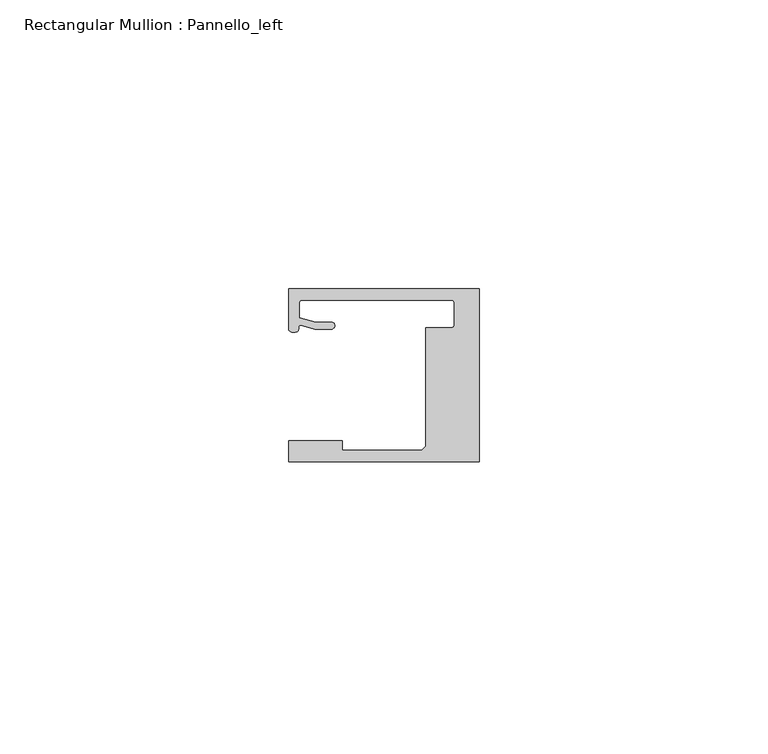
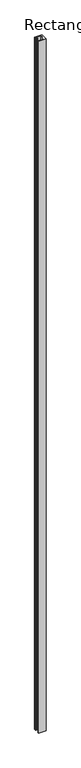
"""IFC4 building model written with IfcOpenShell, lengths in millimetres: member geometry, Rectangular Mullion : Pannello_left."""

from ifc_helpers import new_model, si_unit, frame, origin, place, context, project, spatial, polyline, circle_curve, source, transform, mapped, element, save
from ifc_brep_helpers import plane_surface, cylinder_surface, revolved_surface, extruded_surface, spline_curve, advanced_brep


def rectangular_mullion_pannello_left_2a30ab1a(model_context):
    return source(origin(), model_context, "Body", "AdvancedBrep", [
        advanced_brep(
        [(-33.0, -15.0, 0.0), (0.0, -15.0, 0.0), (0.0, 15.0, 0.0), (-33.0000135, 15.0, 0.0), (-33.0000135, 8.0000472, 0.0), (-30.9223017, 8.6490241, 0.0), (-28.4999305, 7.9999523, 0.0), (-25.59998, 7.9999523, 0.0), (-25.59998, 9.1999523, 0.0), (-28.3419477, 9.1999523, 0.0), (-31.19998, 9.9657591, 0.0), (-31.19998, 12.50001, 0.0), (-30.69998, 13.00001, 0.0), (-4.7999726, 13.00001, 0.0), (-4.2999726, 12.50001, 0.0), (-4.2999726, 8.7500595, 0.0), (-4.7999726, 8.2500595, 0.0), (-9.2999726, 8.2500595, 0.0), (-9.2999726, -12.2999849, 0.0), (-10.0000103, -13.0000004, 0.0), (-23.700041, -13.0000004, 0.0), (-23.700041, -11.3000004, 0.0), (-33.0, -11.3000004, 0.0), (-33.0, -15.0, -3248.9999865), (-33.0, -11.3000004, -3248.9999865), (-23.700041, -11.3000004, -3248.9999865), (-23.700041, -13.0000004, -3248.9999865), (-10.0000103, -13.0000004, -3248.9999865), (-9.2999726, -12.2999849, -3248.9999865), (-9.2999726, 8.2500595, -3248.9999865), (-4.7999726, 8.2500595, -3248.9999865), (-4.2999726, 8.7500595, -3248.9999865), (-4.2999726, 12.50001, -3248.9999865), (-4.7999726, 13.00001, -3248.9999865), (-30.69998, 13.00001, -3248.9999865), (-31.19998, 12.50001, -3248.9999865), (-31.19998, 9.9657591, -3248.9999865), (-28.3419477, 9.1999523, -3248.9999865), (-25.59998, 9.1999523, -3248.9999865), (-25.59998, 7.9999523, -3248.9999865), (-28.4999305, 7.9999523, -3248.9999865), (-30.9223017, 8.6490241, -3248.9999865), (-33.0000135, 8.0000472, -3248.9999865), (-33.0000135, 15.0, -3248.9999865), (0.0, 15.0, -3248.9999865), (0.0, -15.0, -3248.9999865)],
        [
            (0, 1),
            (1, 2),
            (2, 3),
            (3, 4),
            (4, 5, spline_curve(3, [(-33.0000135, 8.0000472, 0.0), (-33.0000135, 7.457047519, 0.0), (-32.262327879, 7.456527435, 0.0), (-31.357433266, 7.563996614, 0.0), (-31.305645054, 7.690065204, 0.0), (-31.298563602, 8.366228555, 0.0), (-31.312054066, 8.717747958, 0.0), (-30.9223017, 8.6490241, 0.0)], [4, 2, 2, 4], [0.0, 0.0027053965905959043, 0.0058611956533709, 0.007702013405570312])),
            (5, 6),
            (6, 7),
            (7, 8, circle_curve(frame((-25.59998, 8.5999523, 0.0), z_axis=(0.0, 0.0, 1.0), x_axis=(0.0, 1.0, 0.0)), 0.6)),
            (8, 9),
            (9, 10),
            (10, 11),
            (11, 12, circle_curve(frame((-30.69998, 12.50001, 0.0), z_axis=(0.0, 0.0, -1.0), x_axis=(0.0, 1.0, 0.0)), 0.5)),
            (12, 13),
            (13, 14, circle_curve(frame((-4.7999726, 12.50001, 0.0), z_axis=(0.0, 0.0, -1.0), x_axis=(1.0, 0.0, 0.0)), 0.5)),
            (14, 15),
            (15, 16, circle_curve(frame((-4.7999726, 8.7500595, 0.0), z_axis=(0.0, 0.0, -1.0), x_axis=(0.0, -1.0, 0.0)), 0.5)),
            (16, 17),
            (17, 18),
            (18, 19),
            (19, 20),
            (20, 21),
            (21, 22),
            (22, 0),
            (23, 24),
            (24, 25),
            (25, 26),
            (26, 27),
            (27, 28),
            (28, 29),
            (29, 30),
            (30, 31, circle_curve(frame((-4.7999726, 8.7500595, -3248.9999865), z_axis=(0.0, 0.0, 1.0), x_axis=(0.0, -1.0, 0.0)), 0.5)),
            (31, 32),
            (32, 33, circle_curve(frame((-4.7999726, 12.50001, -3248.9999865), z_axis=(0.0, 0.0, 1.0), x_axis=(1.0, 0.0, 0.0)), 0.5)),
            (33, 34),
            (34, 35, circle_curve(frame((-30.69998, 12.50001, -3248.9999865), z_axis=(0.0, 0.0, 1.0), x_axis=(0.0, 1.0, 0.0)), 0.5)),
            (35, 36),
            (36, 37),
            (37, 38),
            (38, 39, circle_curve(frame((-25.59998, 8.5999523, -3248.9999865), z_axis=(0.0, 0.0, -1.0), x_axis=(0.0, 1.0, 0.0)), 0.6)),
            (39, 40),
            (40, 41),
            (41, 42, spline_curve(3, [(-30.9223017, 8.6490241, -3248.9999865), (-31.312054066, 8.717747958, -3248.9999865), (-31.298563602, 8.366228555, -3248.9999865), (-31.305645054, 7.690065204, -3248.9999865), (-31.357433266, 7.563996614, -3248.9999865), (-32.262327879, 7.456527435, -3248.9999865), (-33.0000135, 7.457047519, -3248.9999865), (-33.0000135, 8.0000472, -3248.9999865)], [4, 2, 2, 4], [0.0, 0.001840817752199412, 0.004996616814974408, 0.007702013405570312])),
            (42, 43),
            (43, 44),
            (44, 45),
            (45, 23),
            (0, 23),
            (45, 1),
            (44, 2),
            (43, 3),
            (42, 4),
            (41, 5),
            (40, 6),
            (39, 7),
            (38, 8),
            (37, 9),
            (36, 10),
            (35, 11),
            (34, 12),
            (33, 13),
            (32, 14),
            (31, 15),
            (30, 16),
            (29, 17),
            (28, 18),
            (27, 19),
            (26, 20),
            (25, 21),
            (24, 22),
        ],
        [
            plane_surface(frame((0.0, -36.2491502, 0.0), z_axis=(0.0, 0.0, 1.0), x_axis=(-1.0, 0.0, 0.0))),
            plane_surface(frame((0.0, -36.2491502, -3248.9999865), z_axis=(0.0, 0.0, -1.0), x_axis=(-1.0, 0.0, 0.0))),
            plane_surface(frame((-33.0, -15.0, 0.0), z_axis=(0.0, -1.0, 0.0), x_axis=(0.0, 0.0, -1.0))),
            plane_surface(frame((0.0, -15.0, 0.0), z_axis=(1.0, 0.0, 0.0), x_axis=(0.0, 0.0, -1.0))),
            plane_surface(frame((0.0, 15.0, 0.0), z_axis=(0.0, 1.0, 0.0), x_axis=(0.0, 0.0, -1.0))),
            plane_surface(frame((-33.0000135, 15.0, 0.0), z_axis=(-1.0, 0.0, 0.0), x_axis=(0.0, 0.0, -1.0))),
            extruded_surface(spline_curve(3, [(-33.0000135, 8.0000472, -3248.9999865), (-33.0000135, 7.457047519, -3248.9999865), (-32.262327879, 7.456527435, -3248.9999865), (-31.357433266, 7.563996614, -3248.9999865), (-31.305645054, 7.690065204, -3248.9999865), (-31.298563602, 8.366228555, -3248.9999865), (-31.312054066, 8.717747958, -3248.9999865), (-30.9223017, 8.6490241, -3248.9999865)], [4, 2, 2, 4], [0.0, 0.0027053965905959043, 0.0058611956533709, 0.007702013405570312]), (0.0, 0.0, 3248.9999865), 3248.9999865),
            plane_surface(frame((-30.9223017, 8.6490241, 0.0), z_axis=(-0.25881883200192934, -0.9659258833891746, 0.0), x_axis=(0.0, 0.0, -1.0))),
            plane_surface(frame((-28.4999305, 7.9999523, 0.0), z_axis=(0.0, -1.0, 0.0), x_axis=(0.0, 0.0, -1.0))),
            cylinder_surface(frame((-25.59998, 8.5999523, 0.0), z_axis=(0.0, 0.0, 1.0), x_axis=(0.0, 1.0, 0.0)), 0.6),
            plane_surface(frame((-25.59998, 9.1999523, 0.0), z_axis=(0.0, 1.0, 0.0), x_axis=(0.0, 0.0, -1.0))),
            plane_surface(frame((-28.3419477, 9.1999523, 0.0), z_axis=(0.25881883204288636, 0.9659258833782002, 0.0), x_axis=(0.0, 0.0, -1.0))),
            plane_surface(frame((-31.19998, 9.9657591, 0.0), z_axis=(1.0, 0.0, 0.0), x_axis=(0.0, 0.0, -1.0))),
            revolved_surface(polyline([(-30.69998, 13.00001, -3248.9999865), (-30.69998, 13.00001, 0.0)]), (-30.69998, 12.50001, 0.0), (0.0, 0.0, -1.0)),
            plane_surface(frame((-30.69998, 13.00001, 0.0), z_axis=(0.0, -1.0, 0.0), x_axis=(0.0, 0.0, -1.0))),
            revolved_surface(polyline([(-4.2999726, 12.50001, -3248.9999865), (-4.2999726, 12.50001, 0.0)]), (-4.7999726, 12.50001, 0.0), (0.0, 0.0, -1.0)),
            plane_surface(frame((-4.2999726, 12.50001, 0.0), z_axis=(-1.0, 0.0, 0.0), x_axis=(0.0, 0.0, -1.0))),
            revolved_surface(polyline([(-4.7999726, 8.2500595, -3248.9999865), (-4.7999726, 8.2500595, 0.0)]), (-4.7999726, 8.7500595, 0.0), (0.0, 0.0, -1.0)),
            plane_surface(frame((-4.7999726, 8.2500595, 0.0), z_axis=(0.0, 1.0, 0.0), x_axis=(0.0, 0.0, -1.0))),
            plane_surface(frame((-9.2999726, 8.2500595, 0.0), z_axis=(-1.0, 0.0, 0.0), x_axis=(0.0, 0.0, -1.0))),
            plane_surface(frame((-9.2999726, -12.2999849, 0.0), z_axis=(-0.7070955486277984, 0.7071180135668678, 0.0), x_axis=(0.0, 0.0, -1.0))),
            plane_surface(frame((-10.0000103, -13.0000004, 0.0), z_axis=(0.0, 1.0, 0.0), x_axis=(0.0, 0.0, -1.0))),
            plane_surface(frame((-23.700041, -13.0000004, 0.0), z_axis=(1.0, 0.0, 0.0), x_axis=(0.0, 0.0, -1.0))),
            plane_surface(frame((-23.700041, -11.3000004, 0.0), z_axis=(0.0, 1.0, 0.0), x_axis=(0.0, 0.0, -1.0))),
            plane_surface(frame((-33.0, -11.3000004, 0.0), z_axis=(-1.0, 0.0, 0.0), x_axis=(0.0, 0.0, -1.0))),
        ],
        [
            (0, [[1, 2, 3, 4, 5, 6, 7, 8, 9, 10, 11, 12, 13, 14, 15, 16, 17, 18, 19, 20, 21, 22, 23]]),
            (1, [[24, 25, 26, 27, 28, 29, 30, 31, 32, 33, 34, 35, 36, 37, 38, 39, 40, 41, 42, 43, 44, 45, 46]]),
            (2, [[-1, 47, -46, 48]]),
            (3, [[-2, -48, -45, 49]]),
            (4, [[-3, -49, -44, 50]]),
            (5, [[-4, -50, -43, 51]]),
            (6, [[-5, -51, -42, 52]]),
            (7, [[-6, -52, -41, 53]]),
            (8, [[-7, -53, -40, 54]]),
            (9, [[-8, -54, -39, 55]]),
            (10, [[-9, -55, -38, 56]]),
            (11, [[-10, -56, -37, 57]]),
            (12, [[-11, -57, -36, 58]]),
            (13, [[-12, -58, -35, 59]]),
            (14, [[-13, -59, -34, 60]]),
            (15, [[-14, -60, -33, 61]]),
            (16, [[-15, -61, -32, 62]]),
            (17, [[-16, -62, -31, 63]]),
            (18, [[-17, -63, -30, 64]]),
            (19, [[-18, -64, -29, 65]]),
            (20, [[-19, -65, -28, 66]]),
            (21, [[-20, -66, -27, 67]]),
            (22, [[-21, -67, -26, 68]]),
            (23, [[-22, -68, -25, 69]]),
            (24, [[-23, -69, -24, -47]]),
        ],
    ),
    ])


if __name__ == "__main__":
    model = new_model("IFC4")
    model_context = context("Model", 3, world=origin())
    ifc_project = project(units=[si_unit("LENGTHUNIT", "METRE", prefix="MILLI")], contexts=[model_context])
    site = spatial("IfcSite", under=ifc_project)
    building = spatial("IfcBuilding", under=site)
    placement = place(None, origin())
    rectangular_mullion_pannello_left_shape = rectangular_mullion_pannello_left_2a30ab1a(model_context)
    element("IfcMember", 1, ObjectType="Rectangular Mullion : Pannello_left", at=placement, inside=building, context=model_context, shape_type="MappedRepresentation", body=[
        mapped(rectangular_mullion_pannello_left_shape, transform((0.0, 0.0, 0.0), x_axis=(1.0, 0.0, 0.0), y_axis=(0.0, 1.0, 0.0), z_axis=(0.0, 0.0, 1.0))),
    ])
    save(model, "model.ifc")

# Revit data of these elements
# Type "Rectangular Mullion : Pannello_left"
#   built-in parameter 1007322 = 0.0984252 (stored number, unit not read)
#   built-in parameter 1007320 = 0.0305117 (stored number, unit not read)
